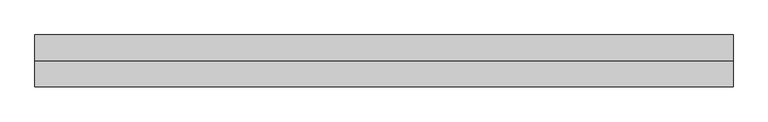
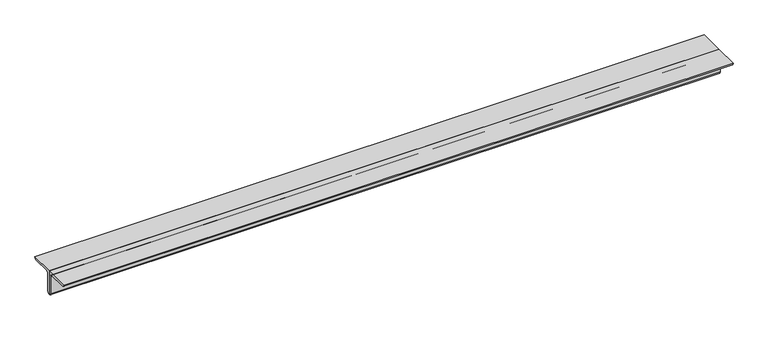
"""IFC4 building model written with IfcOpenShell, lengths in millimetres: member geometry, 0123_Steel Framing_2Ls-KSD3502 : H_SB_AR_S04_2Ls-130x130x12_VBR1."""

import ifcopenshell
import ifcopenshell.guid

model = None  # the IFC model being written
_history = None  # IfcOwnerHistory: only IFC2X3 demands one
_inside = {}  # id of a spatial element -> (the spatial element, [elements in it])
_under = {}  # id of a project, library or spatial element -> (it, [spatial elements below it])
_declared = {}  # id of a project -> (the project, [libraries it declares])
_typed = {}  # id of a type object -> (the type object, [elements of that type])
_made_of = {}  # id of a material, layer set ... -> (it, [elements and type objects made of it])


def new_model(schema):
    """Start an empty IFC model of exactly this schema.

    Asked for "IFC4X3", IfcOpenShell would pick the latest addendum, in which some entities
    have other attributes; the version numbers below select the first issue.
    IFC2X3 requires an IfcOwnerHistory on every rooted entity: one is made here for all.
    """
    global model, _history
    if schema == "IFC4X3":
        model = ifcopenshell.file(schema_version=(4, 3, 0, 0))
    else:
        model = ifcopenshell.file(schema=schema)
    _inside.clear()
    _under.clear()
    _declared.clear()
    _typed.clear()
    _made_of.clear()
    _history = None
    if model.schema == "IFC2X3":
        org = make("IfcOrganization", Name="unknown")
        user = make(
            "IfcPersonAndOrganization",
            ThePerson=make("IfcPerson", FamilyName="unknown"),
            TheOrganization=org,
        )
        app = make(
            "IfcApplication",
            ApplicationDeveloper=org,
            Version="unknown",
            ApplicationFullName="unknown",
            ApplicationIdentifier="unknown",
        )
        _history = make(
            "IfcOwnerHistory",
            OwningUser=user,
            OwningApplication=app,
            ChangeAction="ADDED",
            CreationDate=0,
        )
    return model


def make(cls, **values):
    """One entity of the class cls with the attributes given. An attribute that is None is left unset."""
    return model.create_entity(
        cls, **{name: value for name, value in values.items() if value is not None}
    )


def rooted(cls, **values):
    """An entity with a GlobalId (a new one), such as an element, a storey or a relation."""
    return make(cls, GlobalId=ifcopenshell.guid.new(), OwnerHistory=_history, **values)


def si_unit(unit_type, name, prefix=None):
    """IfcSIUnit, for example si_unit("LENGTHUNIT", "METRE", prefix="MILLI")."""
    return make("IfcSIUnit", UnitType=unit_type, Prefix=prefix, Name=name)


def assignment(units):
    """IfcUnitAssignment: the units of a project."""
    return None if units is None else make("IfcUnitAssignment", Units=units)


def point(xyz):
    """IfcCartesianPoint."""
    return None if xyz is None else make("IfcCartesianPoint", Coordinates=xyz)


def direction(xyz):
    """IfcDirection."""
    return None if xyz is None else make("IfcDirection", DirectionRatios=xyz)


def frame(location, z_axis=None, x_axis=None):
    """IfcAxis2Placement3D, a coordinate frame: its origin and axes. An axis left out is left unset."""
    return make(
        "IfcAxis2Placement3D",
        Location=point(location),
        Axis=direction(z_axis),
        RefDirection=direction(x_axis),
    )


def frame_2d(location, x_axis=None):
    """IfcAxis2Placement2D, a coordinate frame in the plane: its origin and x axis."""
    return make(
        "IfcAxis2Placement2D", Location=point(location), RefDirection=direction(x_axis)
    )


def origin():
    """The frame at (0, 0, 0) with its axes left unset."""
    return frame((0.0, 0.0, 0.0))


def place(relative_to, where):
    """IfcLocalPlacement: puts the frame where relative to a parent placement (None: the world)."""
    return make(
        "IfcLocalPlacement", PlacementRelTo=relative_to, RelativePlacement=where
    )


def context(
    kind, dimensions, precision=None, world=None, true_north=None, identifier=None
):
    """IfcGeometricRepresentationContext, for example the 3D "Model" context."""
    return make(
        "IfcGeometricRepresentationContext",
        ContextIdentifier=identifier,
        ContextType=kind,
        CoordinateSpaceDimension=dimensions,
        Precision=precision,
        WorldCoordinateSystem=world,
        TrueNorth=true_north,
    )


def project(units=None, contexts=None):
    """IfcProject with its units and contexts."""
    return rooted(
        "IfcProject",
        Name="project",
        RepresentationContexts=contexts,
        UnitsInContext=assignment(units),
    )


def spatial(cls, under=None, at=None, **own):
    """A site, building, storey or space (cls), placed at a placement, below another one or the project."""
    s = rooted(cls, ObjectPlacement=at, **own)
    if under is not None:
        _under.setdefault(under.id(), (under, []))[1].append(s)
    return s


def polyline(points):
    """IfcPolyline through the points."""
    return make("IfcPolyline", Points=[point(p) for p in points])


def circle_curve(where, radius):
    """IfcCircle in the frame where."""
    return make("IfcCircle", Position=where, Radius=radius)


def trimmed(basis, trim1, trim2, sense, master):
    """IfcTrimmedCurve: the piece of a basis curve between two trims."""
    return make(
        "IfcTrimmedCurve",
        BasisCurve=basis,
        Trim1=trim1,
        Trim2=trim2,
        SenseAgreement=sense,
        MasterRepresentation=master,
    )


def segment(curve, same_sense, transition):
    """IfcCompositeCurveSegment."""
    return make(
        "IfcCompositeCurveSegment",
        Transition=transition,
        SameSense=same_sense,
        ParentCurve=curve,
    )


def composite_curve(segments, self_intersect=None):
    """IfcCompositeCurve: segments joined end to end."""
    return make("IfcCompositeCurve", Segments=segments, SelfIntersect=self_intersect)


def outline(outer, holes=None, kind="AREA"):
    """IfcArbitraryClosedProfileDef: a profile drawn as a closed curve; with holes, ...WithVoids."""
    if holes is None:
        return make("IfcArbitraryClosedProfileDef", ProfileType=kind, OuterCurve=outer)
    return make(
        "IfcArbitraryProfileDefWithVoids",
        ProfileType=kind,
        OuterCurve=outer,
        InnerCurves=holes,
    )


def extrude(swept, where, along, depth):
    """IfcExtrudedAreaSolid: the profile swept, set in the frame where, extruded along a direction by depth."""
    return make(
        "IfcExtrudedAreaSolid",
        SweptArea=swept,
        Position=where,
        ExtrudedDirection=direction(along),
        Depth=depth,
    )


def shape(context_of_items, identifier, shape_type, items):
    """IfcShapeRepresentation: the items that make up one representation, for example the "Body"."""
    return make(
        "IfcShapeRepresentation",
        ContextOfItems=context_of_items,
        RepresentationIdentifier=identifier,
        RepresentationType=shape_type,
        Items=items,
    )


def source(mapping_origin, context_of_items, identifier, shape_type, items):
    """IfcRepresentationMap: a shape defined once, which mapped items show again and again."""
    return make(
        "IfcRepresentationMap",
        MappingOrigin=mapping_origin,
        MappedRepresentation=shape(context_of_items, identifier, shape_type, items),
    )


def transform(
    local_origin,
    x_axis=None,
    y_axis=None,
    z_axis=None,
    scale=None,
    scale2=None,
    scale3=None,
    uniform=True,
):
    """IfcCartesianTransformationOperator3D, or its non-uniform kind. x_axis, y_axis, z_axis: its Axis1, 2, 3."""
    if uniform:
        return make(
            "IfcCartesianTransformationOperator3D",
            Axis1=direction(x_axis),
            Axis2=direction(y_axis),
            LocalOrigin=point(local_origin),
            Scale=scale,
            Axis3=direction(z_axis),
        )
    return make(
        "IfcCartesianTransformationOperator3DnonUniform",
        Axis1=direction(x_axis),
        Axis2=direction(y_axis),
        LocalOrigin=point(local_origin),
        Scale=scale,
        Axis3=direction(z_axis),
        Scale2=scale2,
        Scale3=scale3,
    )


def mapped(mapping_source, mapping_target):
    """IfcMappedItem: shows the shape of a source again, moved by a transform."""
    return make(
        "IfcMappedItem", MappingSource=mapping_source, MappingTarget=mapping_target
    )


def made_of(thing, what):
    """Note that an element or type object is made of a material, layer set ...; save() writes the relation."""
    if what is not None:
        _made_of.setdefault(what.id(), (what, []))[1].append(thing)
    return thing


def element(
    cls,
    number,
    at=None,
    inside=None,
    cuts=None,
    type_object=None,
    material=None,
    context=None,
    identifier="Body",
    shape_type=None,
    held_by="IfcProductDefinitionShape",
    body=None,
    shapes=None,
    **own,
):
    """One element of the class cls, such as IfcWall. Its Tag is "e" and its number.

    at: its placement. inside: the storey or other place that contains it. cuts: it is an
    opening in that element (IfcRelVoidsElement). A single representation is given by context,
    identifier, shape_type and body (its items); several are given by shapes. held_by: the class
    of the entity that holds the representations. save() writes the other relations.
    """
    e = rooted(cls, Tag="e%d" % number, ObjectPlacement=at, **own)
    if body is not None:
        shapes = [shape(context, identifier, shape_type, body)]
    if shapes is not None:
        e.Representation = make(held_by, Representations=shapes)
    if inside is not None:
        _inside.setdefault(inside.id(), (inside, []))[1].append(e)
    if cuts is not None:
        rooted(
            "IfcRelVoidsElement", RelatingBuildingElement=cuts, RelatedOpeningElement=e
        )
    if type_object is not None:
        _typed.setdefault(type_object.id(), (type_object, []))[1].append(e)
    return made_of(e, material)


def aggregate(whole, parts):
    """IfcRelAggregates: a whole, such as a stair, and the parts it consists of."""
    return rooted("IfcRelAggregates", RelatingObject=whole, RelatedObjects=parts)


def save(model, path):
    """Write the relations noted so far, then the file.

    IfcRelAggregates (storeys below a building ...), IfcRelContainedInSpatialStructure (elements
    in a storey), IfcRelDefinesByType, IfcRelAssociatesMaterial and IfcRelDeclares: one each for
    every whole, place, type object, material and project.
    """
    for whole, parts in _under.values():
        aggregate(whole, parts)
    for where, things in _inside.values():
        rooted(
            "IfcRelContainedInSpatialStructure",
            RelatedElements=things,
            RelatingStructure=where,
        )
    for kind, things in _typed.values():
        rooted("IfcRelDefinesByType", RelatedObjects=things, RelatingType=kind)
    for what, things in _made_of.values():
        rooted("IfcRelAssociatesMaterial", RelatedObjects=things, RelatingMaterial=what)
    for by, libraries in _declared.values():
        rooted("IfcRelDeclares", RelatingContext=by, RelatedDefinitions=libraries)
    model.write(path)


def member_96e87236(model_context):
    return source(origin(), model_context, "Body", "SweptSolid", [
        extrude(outline(composite_curve([segment(polyline([(0.0, 36.4), (130.0, 36.4)]), True, "CONTINUOUS"), segment(trimmed(circle_curve(frame_2d((118.0, 36.4)), 12.0), [point((130.0, 36.4))], [point((118.0, 24.4))], False, "CARTESIAN"), True, "CONTINUOUS"), segment(polyline([(118.0, 24.4), (24.0, 24.4)]), True, "CONTINUOUS"), segment(trimmed(circle_curve(frame_2d((24.0, 12.4)), 12.0), [point((24.0, 24.4))], [point((12.0, 12.4))], True, "CARTESIAN"), True, "CONTINUOUS"), segment(polyline([(12.0, 12.4), (12.0, -81.6)]), True, "CONTINUOUS"), segment(trimmed(circle_curve(frame_2d((0.0, -81.6)), 12.0), [point((12.0, -81.6))], [point((0.0, -93.6))], False, "CARTESIAN"), True, "CONTINUOUS"), segment(polyline([(0.0, -93.6), (0.0, 36.4)]), True, "CONTINUOUS")], self_intersect=False)), frame((-1749.149537, 0.0, 0.0), z_axis=(1.0, 0.0, 0.0), x_axis=(0.0, 1.0, 0.0)), (0.0, 0.0, 1.0), 3498.299074),
        extrude(outline(composite_curve([segment(polyline([(0.0, 36.4), (0.0, -93.6)]), True, "CONTINUOUS"), segment(trimmed(circle_curve(frame_2d((0.0, -81.6)), 12.0), [point((0.0, -93.6))], [point((-12.0, -81.6))], False, "CARTESIAN"), True, "CONTINUOUS"), segment(polyline([(-12.0, -81.6), (-12.0, 12.4)]), True, "CONTINUOUS"), segment(trimmed(circle_curve(frame_2d((-24.0, 12.4)), 12.0), [point((-12.0, 12.4))], [point((-24.0, 24.4))], True, "CARTESIAN"), True, "CONTINUOUS"), segment(polyline([(-24.0, 24.4), (-118.0, 24.4)]), True, "CONTINUOUS"), segment(trimmed(circle_curve(frame_2d((-118.0, 36.4)), 12.0), [point((-118.0, 24.4))], [point((-130.0, 36.4))], False, "CARTESIAN"), True, "CONTINUOUS"), segment(polyline([(-130.0, 36.4), (0.0, 36.4)]), True, "CONTINUOUS")], self_intersect=False)), frame((-1749.149537, 0.0, 0.0), z_axis=(1.0, 0.0, 0.0), x_axis=(0.0, 1.0, 0.0)), (0.0, 0.0, 1.0), 3498.299074),
    ])


if __name__ == "__main__":
    model = new_model("IFC4")
    model_context = context("Model", 3, world=origin())
    ifc_project = project(units=[si_unit("LENGTHUNIT", "METRE", prefix="MILLI")], contexts=[model_context])
    site = spatial("IfcSite", under=ifc_project)
    building = spatial("IfcBuilding", under=site)
    placement = place(None, origin())
    member_shape = member_96e87236(model_context)
    element("IfcMember", 1, ObjectType="0123_Steel Framing_2Ls-KSD3502 : H_SB_AR_S04_2Ls-130x130x12_VBR1", at=placement, inside=building, context=model_context, shape_type="MappedRepresentation", body=[
        mapped(member_shape, transform((0.0, 0.0, 0.0), x_axis=(1.0, 0.0, 0.0), y_axis=(0.0, 1.0, 0.0), z_axis=(0.0, 0.0, 1.0))),
    ])
    save(model, "model.ifc")

# Revit data of these elements
# Type "0123_Steel Framing_2Ls-KSD3502 : H_SB_AR_S04_2Ls-130x130x12_VBR1"
#   Assembly Code = "B10"
#   Legs = "SLBB"
#   W = 8.97
#   Perimeter = 1.04 m²/m
#   Nominal Weight = 46.80 kgf/m
#   Length [instance default] = 1000 mm
#   Space = 0 mm
#   b = 130 mm
#   d = 130 mm
#   t = 12 mm
#   y = 36.4 mm
#   A = 0.005952 m²
#   Structural Material [instance default] = Steel ASTM A36
# Element 1 (IfcMember, "0123_Steel Framing_2Ls-KSD3502 : H_SB_AR_S04_2Ls-130x130x12_VBR1")
#   Structural Material = Steel, 45-345
#   Materials on its faces: "Steel, 45-345"
# Materials
#   "Steel ASTM A36": class "Metal", colour RGB 199 199 199, transparency 0, Description = "Structural steel, ASTM A36 Grade B, mill finish", Cost = 0
#   "Steel, 45-345": class "Metal", colour RGB 189 187 185, transparency 0, Description = "Steel 345 MPa", Cost = 0
